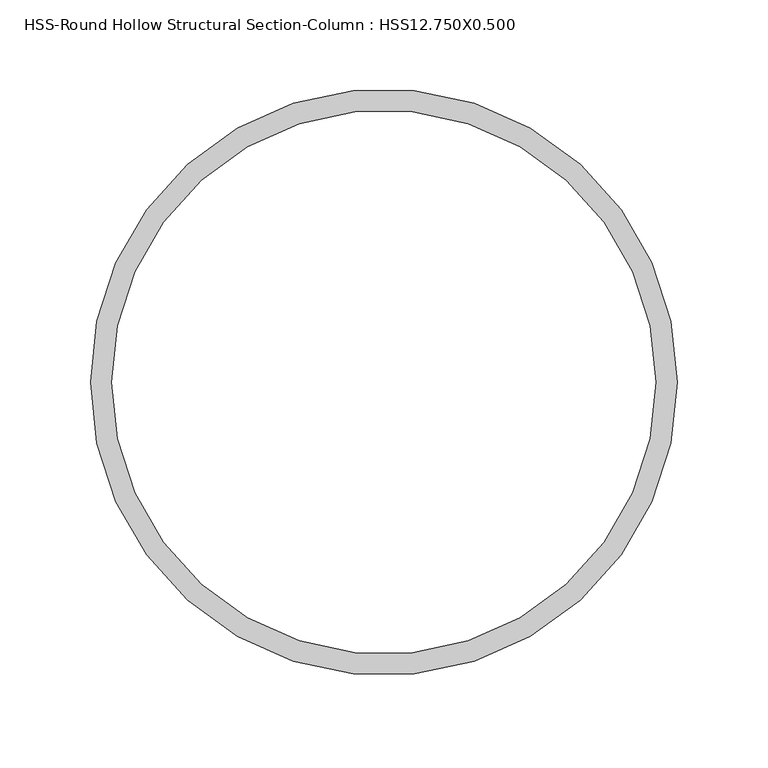
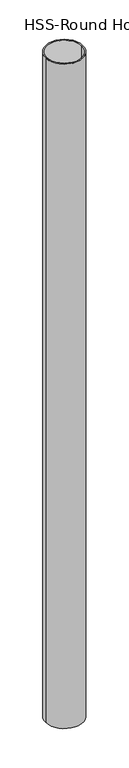
"""IFC4 building model written with IfcOpenShell, lengths in millimetres: column geometry, HSS-Round Hollow Structural Section-Column : HSS12.750X0.500."""

from ifc_helpers import new_model, si_unit, point, frame, origin, origin_2d, place, context, project, spatial, circle_curve, trimmed, segment, composite_curve, outline, extrude, source, transform, mapped, element, save


def hss_round_hollow_structural_section_column_hss12_750x0_500_3b49a283(model_context):
    return source(origin(), model_context, "Body", "SweptSolid", [
        extrude(outline(composite_curve([segment(trimmed(circle_curve(origin_2d(), 161.925), [point((-161.925, 0.0))], [point((161.925, 0.0))], False, "CARTESIAN"), True, "CONTINUOUS"), segment(trimmed(circle_curve(origin_2d(), 161.925), [point((161.925, 0.0))], [point((-161.925, 0.0))], False, "CARTESIAN"), True, "CONTINUOUS")], self_intersect=False), holes=[composite_curve([segment(trimmed(circle_curve(origin_2d(), 150.114), [point((-150.114, 0.0))], [point((150.114, 0.0))], True, "CARTESIAN"), True, "CONTINUOUS"), segment(trimmed(circle_curve(origin_2d(), 150.114), [point((150.114, 0.0))], [point((-150.114, 0.0))], True, "CARTESIAN"), True, "CONTINUOUS")], self_intersect=False)]), frame((0.0, 0.0, 5969.0), z_axis=(0.0, 0.0, 1.0), x_axis=(1.0, 0.0, 0.0)), (0.0, 0.0, 1.0), 6096.0),
    ])


if __name__ == "__main__":
    model = new_model("IFC4")
    model_context = context("Model", 3, world=origin())
    ifc_project = project(units=[si_unit("LENGTHUNIT", "METRE", prefix="MILLI")], contexts=[model_context])
    site = spatial("IfcSite", under=ifc_project)
    building = spatial("IfcBuilding", under=site)
    placement = place(None, origin())
    hss_round_hollow_structural_section_column_hss12_750x0_500_shape = hss_round_hollow_structural_section_column_hss12_750x0_500_3b49a283(model_context)
    element("IfcColumn", 1, ObjectType="HSS-Round Hollow Structural Section-Column : HSS12.750X0.500", at=placement, inside=building, context=model_context, shape_type="MappedRepresentation", body=[
        mapped(hss_round_hollow_structural_section_column_hss12_750x0_500_shape, transform((0.0, 0.0, 0.0), x_axis=(1.0, 0.0, 0.0), y_axis=(0.0, 1.0, 0.0), z_axis=(0.0, 0.0, 1.0))),
    ])
    save(model, "model.ifc")

# Revit data of these elements
# Type "HSS-Round Hollow Structural Section-Column : HSS12.750X0.500"
#   Assembly Code = "B10"
#   W = 65.5
#   OD = 1' - 0 3/4"
#   t = 0' - 0.465"
#   A = 0.124306 SF
#   Column Material [instance default] = Metal - Steel - ASTM A53
# Element 1 (IfcColumn, "HSS-Round Hollow Structural Section-Column : HSS12.750X0.500")
#   Materials on its faces: "Metal - Steel - ASTM A53"
# Materials
#   "Metal - Steel - ASTM A53": class "Metal", colour RGB 128 0 0, transparency 0
